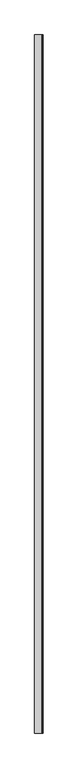
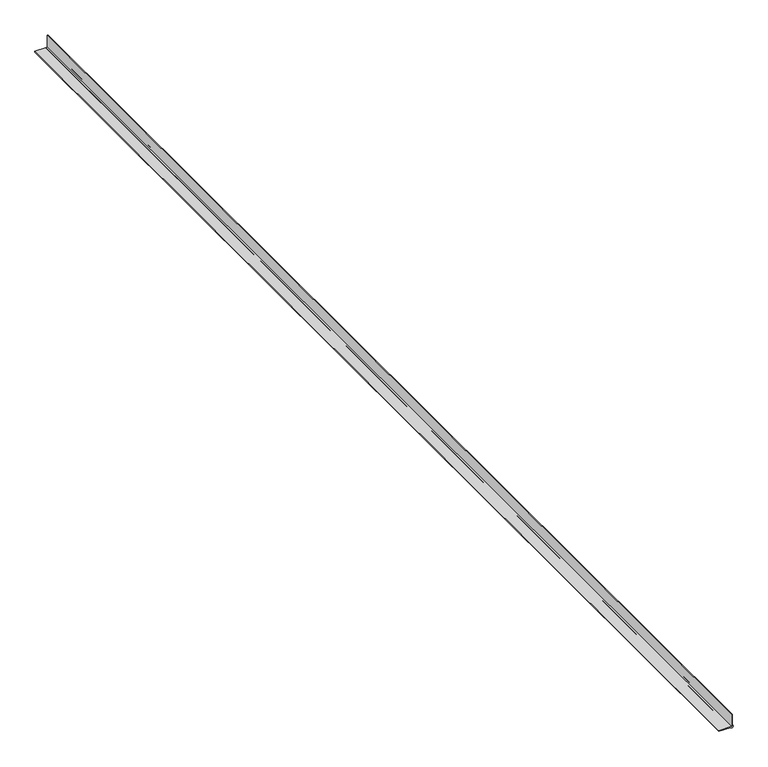
"""IFC4 building model written with IfcOpenShell, lengths in millimetres: proxy geometry, Blocking084 4:Blocking084 10484:304629 : Blocking084 4:Blocking084 10484:304629."""

from ifc_helpers import new_model, si_unit, point, frame, frame_2d, origin, place, context, project, spatial, polyline, circle_curve, trimmed, segment, composite_curve, outline, extrude, source, transform, mapped, element, save


def generic_models_8d55ade1(model_context):
    return source(origin(), model_context, "Body", "SweptSolid", [
        extrude(outline(composite_curve([segment(polyline([(42140.2658547, 10989.7478388), (42140.2658547, 10988.4678388), (42119.1126708, 10988.4678388), (42119.1126708, 10967.3146549), (42117.8326708, 10967.3146549), (42117.8326708, 10986.1661839)]), True, "CONTINUOUS"), segment(trimmed(circle_curve(frame_2d((42119.1126708, 10988.4678388)), 2.6336316), [point((42117.8326708, 10986.1661839))], [point((42121.4143257, 10989.7478388))], False, "CARTESIAN"), True, "CONTINUOUS"), segment(polyline([(42121.4143257, 10989.7478388), (42140.2658547, 10989.7478388)]), True, "CONTINUOUS")], self_intersect=False)), frame((0.0, -774.5586951, 0.0), z_axis=(0.0, 1.0, 0.0), x_axis=(0.0, 0.0, 1.0)), (0.0, 0.0, 1.0), 2000.0),
    ])


if __name__ == "__main__":
    model = new_model("IFC4")
    model_context = context("Model", 3, world=origin())
    ifc_project = project(units=[si_unit("LENGTHUNIT", "METRE", prefix="MILLI")], contexts=[model_context])
    site = spatial("IfcSite", under=ifc_project)
    building = spatial("IfcBuilding", under=site)
    placement = place(None, origin())
    generic_models_shape = generic_models_8d55ade1(model_context)
    element("IfcBuildingElementProxy", 1, Name="Blocking084 4:Blocking084 10484:304629 : Blocking084 4:Blocking084 10484:304629", ObjectType="Blocking084 4:Blocking084 10484:304629 : Blocking084 4:Blocking084 10484:304629", at=placement, inside=building, context=model_context, shape_type="MappedRepresentation", body=[
        mapped(generic_models_shape, transform((0.0, 0.0, 0.0), x_axis=(1.0, 0.0, 0.0), y_axis=(0.0, 1.0, 0.0), z_axis=(0.0, 0.0, 1.0))),
    ])
    save(model, "model.ifc")

# Revit data of these elements
# Type "Blocking084 4:Blocking084 10484:304629 : Blocking084 4:Blocking084 10484:304629"
#   NameOverride = "Blocking084 4:Blocking084 10484:304629"
#   ObjectTypeOverride = "Blocking084 4:Blocking084 10484"
#   Reference = "Blocking084 10484"
#   Category = "Generic Models"
#   Tag = "304629"
# Element 1 (IfcBuildingElementProxy, "Blocking084 4:Blocking084 10484:304629 : Blocking084 4:Blocking084 10484:304629")
#   Materials on its faces: "CORNER BEAD"
# Materials
#   "CORNER BEAD": class "Unassigned", colour RGB 253 236 176, transparency 0, Cost = 0
